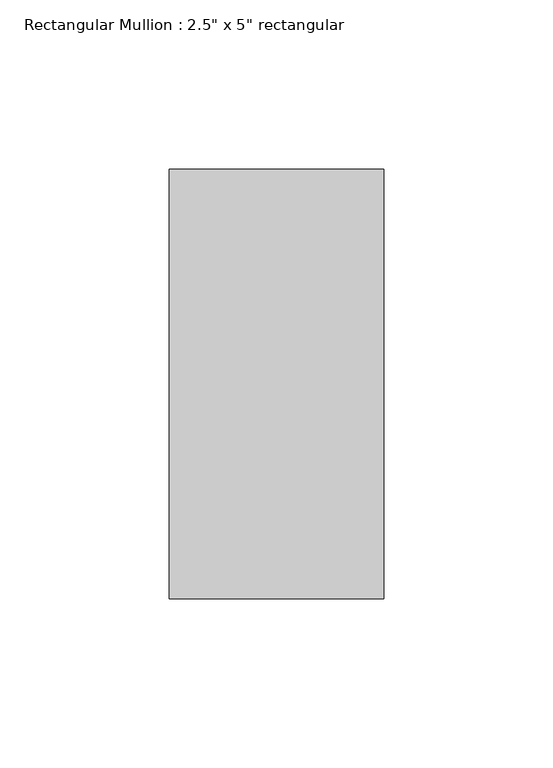
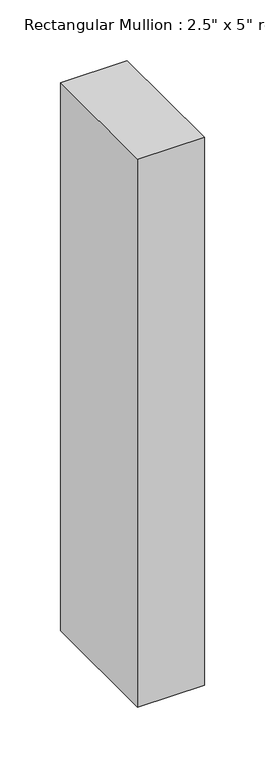
"""IFC4 building model written with IfcOpenShell, lengths in millimetres: member geometry."""

from ifc_helpers import new_model, si_unit, frame, origin, place, context, project, spatial, polyline, outline, extrude, source, transform, mapped, element, save


def member_76b76db9(model_context):
    return source(origin(), model_context, "Body", "SweptSolid", [
        extrude(outline(polyline([(31.75, 63.5), (31.75, -63.5), (-31.75, -63.5), (-31.75, 63.5), (31.75, 63.5)])), frame((0.0, 0.0, -551.035953), z_axis=(0.0, 0.0, 1.0), x_axis=(1.0, 0.0, 0.0)), (0.0, 0.0, 1.0), 551.035953),
    ])


if __name__ == "__main__":
    model = new_model("IFC4")
    model_context = context("Model", 3, world=origin())
    ifc_project = project(units=[si_unit("LENGTHUNIT", "METRE", prefix="MILLI")], contexts=[model_context])
    site = spatial("IfcSite", under=ifc_project)
    building = spatial("IfcBuilding", under=site)
    placement = place(None, origin())
    member_shape = member_76b76db9(model_context)
    element("IfcMember", 1, ObjectType="Rectangular Mullion : 2.5\" x 5\" rectangular", at=placement, inside=building, context=model_context, shape_type="MappedRepresentation", body=[
        mapped(member_shape, transform((0.0, 0.0, 0.0), x_axis=(1.0, 0.0, 0.0), y_axis=(0.0, 1.0, 0.0), z_axis=(0.0, 0.0, 1.0))),
    ])
    save(model, "model.ifc")

# Revit data of these elements
# Type "Rectangular Mullion : 2.5\" x 5\" rectangular"
#   built-in parameter 1007304 = 0.416667 (stored number, unit not read)
#   built-in parameter 1007301 = 0.104167 (stored number, unit not read)
#   built-in parameter 1007300 = 0.104167 (stored number, unit not read)
# Element 1 (IfcMember, "Rectangular Mullion : 2.5\" x 5\" rectangular")
#   Materials on its faces: "Metal - Aluminum 2"
# Materials
#   "Metal - Aluminum 2": class "Metal", colour RGB 189 187 185, transparency 0
